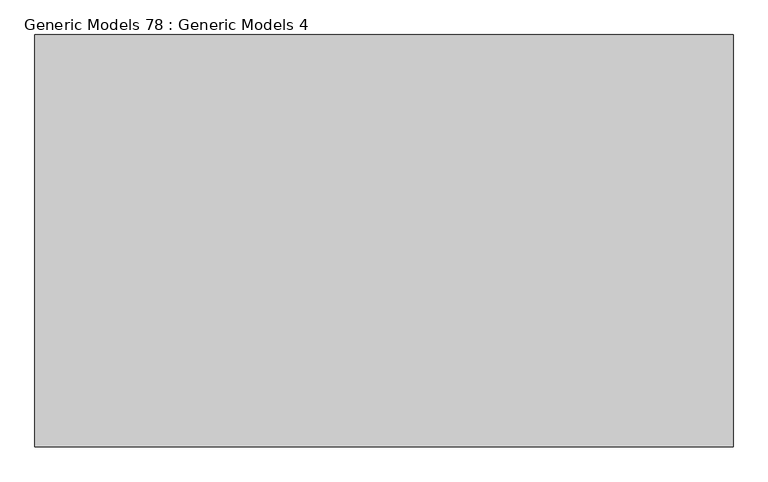
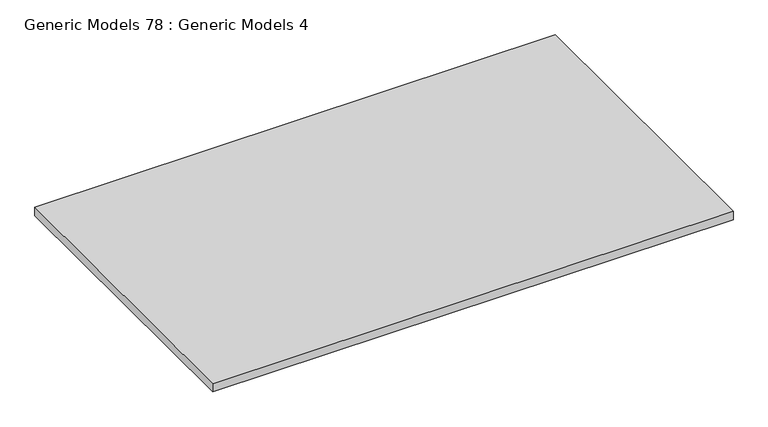
"""IFC4 building model written with IfcOpenShell, lengths in millimetres: proxy geometry, Generic Models 78 : Generic Models 4."""

from ifc_helpers import new_model, si_unit, frame, origin, place, context, project, spatial, polyline, outline, extrude, source, transform, mapped, element, save


def generic_models_78_generic_models_4_fb95c183(model_context):
    return source(origin(), model_context, "Body", "SweptSolid", [
        extrude(outline(polyline([(29256.3806153, -7845.1058743), (29256.3806153, -11442.9554199), (23168.0573109, -11442.9554199), (23168.0573109, -7845.1058743), (29256.3806153, -7845.1058743)])), frame((0.0, 0.0, 122955.6484874), z_axis=(0.0, 0.0, 1.0), x_axis=(1.0, 0.0, 0.0)), (0.0, 0.0, 1.0), 101.6),
    ])


if __name__ == "__main__":
    model = new_model("IFC4")
    model_context = context("Model", 3, world=origin())
    ifc_project = project(units=[si_unit("LENGTHUNIT", "METRE", prefix="MILLI")], contexts=[model_context])
    site = spatial("IfcSite", under=ifc_project)
    building = spatial("IfcBuilding", under=site)
    placement = place(None, origin())
    generic_models_78_generic_models_4_shape = generic_models_78_generic_models_4_fb95c183(model_context)
    element("IfcBuildingElementProxy", 1, Name="Generic Models 78 : Generic Models 4", ObjectType="Generic Models 78 : Generic Models 4", at=placement, inside=building, context=model_context, shape_type="MappedRepresentation", body=[
        mapped(generic_models_78_generic_models_4_shape, transform((0.0, 0.0, 0.0), x_axis=(1.0, 0.0, 0.0), y_axis=(0.0, 1.0, 0.0), z_axis=(0.0, 0.0, 1.0))),
    ])
    save(model, "model.ifc")

# Revit data of these elements
# Element 1 (IfcBuildingElementProxy, "Generic Models 78 : Generic Models 4")
#   Materials on its faces: "_4\" MIN. CRUSHED GRAVEL (NO FINES)"
# Materials
#   "_4\" MIN. CRUSHED GRAVEL (NO FINES)": class "Generic", colour RGB 122 131 148, transparency 0, Cost = 0
